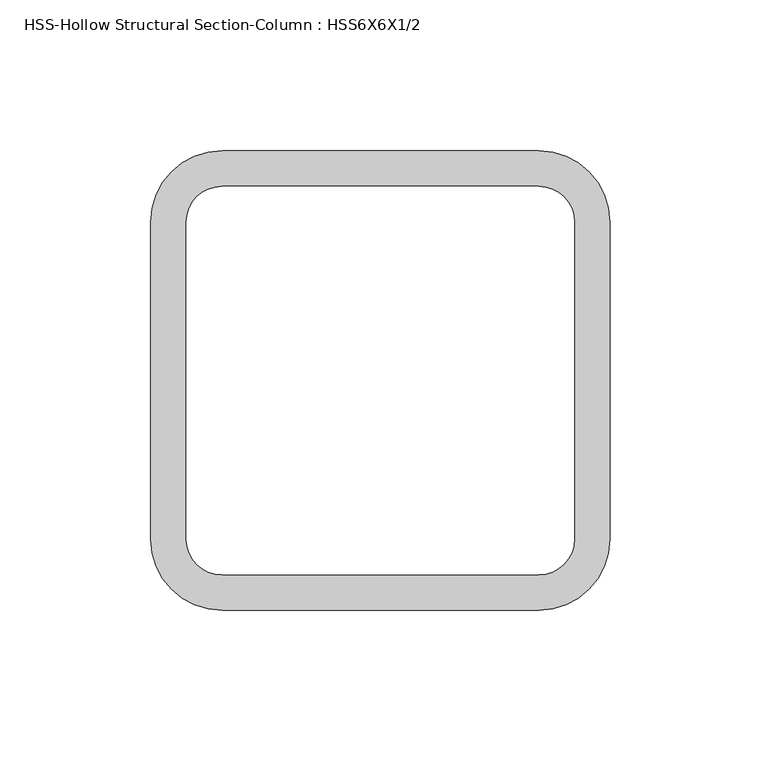
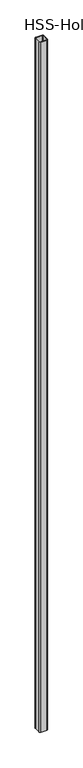
"""IFC4 building model written with IfcOpenShell, lengths in millimetres: column geometry, HSS-Hollow Structural Section-Column : HSS6X6X1/2."""

import ifcopenshell
import ifcopenshell.guid

model = None  # the IFC model being written
_history = None  # IfcOwnerHistory: only IFC2X3 demands one
_inside = {}  # id of a spatial element -> (the spatial element, [elements in it])
_under = {}  # id of a project, library or spatial element -> (it, [spatial elements below it])
_declared = {}  # id of a project -> (the project, [libraries it declares])
_typed = {}  # id of a type object -> (the type object, [elements of that type])
_made_of = {}  # id of a material, layer set ... -> (it, [elements and type objects made of it])


def new_model(schema):
    """Start an empty IFC model of exactly this schema.

    Asked for "IFC4X3", IfcOpenShell would pick the latest addendum, in which some entities
    have other attributes; the version numbers below select the first issue.
    IFC2X3 requires an IfcOwnerHistory on every rooted entity: one is made here for all.
    """
    global model, _history
    if schema == "IFC4X3":
        model = ifcopenshell.file(schema_version=(4, 3, 0, 0))
    else:
        model = ifcopenshell.file(schema=schema)
    _inside.clear()
    _under.clear()
    _declared.clear()
    _typed.clear()
    _made_of.clear()
    _history = None
    if model.schema == "IFC2X3":
        org = make("IfcOrganization", Name="unknown")
        user = make(
            "IfcPersonAndOrganization",
            ThePerson=make("IfcPerson", FamilyName="unknown"),
            TheOrganization=org,
        )
        app = make(
            "IfcApplication",
            ApplicationDeveloper=org,
            Version="unknown",
            ApplicationFullName="unknown",
            ApplicationIdentifier="unknown",
        )
        _history = make(
            "IfcOwnerHistory",
            OwningUser=user,
            OwningApplication=app,
            ChangeAction="ADDED",
            CreationDate=0,
        )
    return model


def make(cls, **values):
    """One entity of the class cls with the attributes given. An attribute that is None is left unset."""
    return model.create_entity(
        cls, **{name: value for name, value in values.items() if value is not None}
    )


def rooted(cls, **values):
    """An entity with a GlobalId (a new one), such as an element, a storey or a relation."""
    return make(cls, GlobalId=ifcopenshell.guid.new(), OwnerHistory=_history, **values)


def si_unit(unit_type, name, prefix=None):
    """IfcSIUnit, for example si_unit("LENGTHUNIT", "METRE", prefix="MILLI")."""
    return make("IfcSIUnit", UnitType=unit_type, Prefix=prefix, Name=name)


def assignment(units):
    """IfcUnitAssignment: the units of a project."""
    return None if units is None else make("IfcUnitAssignment", Units=units)


def point(xyz):
    """IfcCartesianPoint."""
    return None if xyz is None else make("IfcCartesianPoint", Coordinates=xyz)


def direction(xyz):
    """IfcDirection."""
    return None if xyz is None else make("IfcDirection", DirectionRatios=xyz)


def frame(location, z_axis=None, x_axis=None):
    """IfcAxis2Placement3D, a coordinate frame: its origin and axes. An axis left out is left unset."""
    return make(
        "IfcAxis2Placement3D",
        Location=point(location),
        Axis=direction(z_axis),
        RefDirection=direction(x_axis),
    )


def frame_2d(location, x_axis=None):
    """IfcAxis2Placement2D, a coordinate frame in the plane: its origin and x axis."""
    return make(
        "IfcAxis2Placement2D", Location=point(location), RefDirection=direction(x_axis)
    )


def origin():
    """The frame at (0, 0, 0) with its axes left unset."""
    return frame((0.0, 0.0, 0.0))


def place(relative_to, where):
    """IfcLocalPlacement: puts the frame where relative to a parent placement (None: the world)."""
    return make(
        "IfcLocalPlacement", PlacementRelTo=relative_to, RelativePlacement=where
    )


def context(
    kind, dimensions, precision=None, world=None, true_north=None, identifier=None
):
    """IfcGeometricRepresentationContext, for example the 3D "Model" context."""
    return make(
        "IfcGeometricRepresentationContext",
        ContextIdentifier=identifier,
        ContextType=kind,
        CoordinateSpaceDimension=dimensions,
        Precision=precision,
        WorldCoordinateSystem=world,
        TrueNorth=true_north,
    )


def project(units=None, contexts=None):
    """IfcProject with its units and contexts."""
    return rooted(
        "IfcProject",
        Name="project",
        RepresentationContexts=contexts,
        UnitsInContext=assignment(units),
    )


def spatial(cls, under=None, at=None, **own):
    """A site, building, storey or space (cls), placed at a placement, below another one or the project."""
    s = rooted(cls, ObjectPlacement=at, **own)
    if under is not None:
        _under.setdefault(under.id(), (under, []))[1].append(s)
    return s


def polyline(points):
    """IfcPolyline through the points."""
    return make("IfcPolyline", Points=[point(p) for p in points])


def circle_curve(where, radius):
    """IfcCircle in the frame where."""
    return make("IfcCircle", Position=where, Radius=radius)


def trimmed(basis, trim1, trim2, sense, master):
    """IfcTrimmedCurve: the piece of a basis curve between two trims."""
    return make(
        "IfcTrimmedCurve",
        BasisCurve=basis,
        Trim1=trim1,
        Trim2=trim2,
        SenseAgreement=sense,
        MasterRepresentation=master,
    )


def segment(curve, same_sense, transition):
    """IfcCompositeCurveSegment."""
    return make(
        "IfcCompositeCurveSegment",
        Transition=transition,
        SameSense=same_sense,
        ParentCurve=curve,
    )


def composite_curve(segments, self_intersect=None):
    """IfcCompositeCurve: segments joined end to end."""
    return make("IfcCompositeCurve", Segments=segments, SelfIntersect=self_intersect)


def outline(outer, holes=None, kind="AREA"):
    """IfcArbitraryClosedProfileDef: a profile drawn as a closed curve; with holes, ...WithVoids."""
    if holes is None:
        return make("IfcArbitraryClosedProfileDef", ProfileType=kind, OuterCurve=outer)
    return make(
        "IfcArbitraryProfileDefWithVoids",
        ProfileType=kind,
        OuterCurve=outer,
        InnerCurves=holes,
    )


def extrude(swept, where, along, depth):
    """IfcExtrudedAreaSolid: the profile swept, set in the frame where, extruded along a direction by depth."""
    return make(
        "IfcExtrudedAreaSolid",
        SweptArea=swept,
        Position=where,
        ExtrudedDirection=direction(along),
        Depth=depth,
    )


def shape(context_of_items, identifier, shape_type, items):
    """IfcShapeRepresentation: the items that make up one representation, for example the "Body"."""
    return make(
        "IfcShapeRepresentation",
        ContextOfItems=context_of_items,
        RepresentationIdentifier=identifier,
        RepresentationType=shape_type,
        Items=items,
    )


def source(mapping_origin, context_of_items, identifier, shape_type, items):
    """IfcRepresentationMap: a shape defined once, which mapped items show again and again."""
    return make(
        "IfcRepresentationMap",
        MappingOrigin=mapping_origin,
        MappedRepresentation=shape(context_of_items, identifier, shape_type, items),
    )


def transform(
    local_origin,
    x_axis=None,
    y_axis=None,
    z_axis=None,
    scale=None,
    scale2=None,
    scale3=None,
    uniform=True,
):
    """IfcCartesianTransformationOperator3D, or its non-uniform kind. x_axis, y_axis, z_axis: its Axis1, 2, 3."""
    if uniform:
        return make(
            "IfcCartesianTransformationOperator3D",
            Axis1=direction(x_axis),
            Axis2=direction(y_axis),
            LocalOrigin=point(local_origin),
            Scale=scale,
            Axis3=direction(z_axis),
        )
    return make(
        "IfcCartesianTransformationOperator3DnonUniform",
        Axis1=direction(x_axis),
        Axis2=direction(y_axis),
        LocalOrigin=point(local_origin),
        Scale=scale,
        Axis3=direction(z_axis),
        Scale2=scale2,
        Scale3=scale3,
    )


def mapped(mapping_source, mapping_target):
    """IfcMappedItem: shows the shape of a source again, moved by a transform."""
    return make(
        "IfcMappedItem", MappingSource=mapping_source, MappingTarget=mapping_target
    )


def made_of(thing, what):
    """Note that an element or type object is made of a material, layer set ...; save() writes the relation."""
    if what is not None:
        _made_of.setdefault(what.id(), (what, []))[1].append(thing)
    return thing


def element(
    cls,
    number,
    at=None,
    inside=None,
    cuts=None,
    type_object=None,
    material=None,
    context=None,
    identifier="Body",
    shape_type=None,
    held_by="IfcProductDefinitionShape",
    body=None,
    shapes=None,
    **own,
):
    """One element of the class cls, such as IfcWall. Its Tag is "e" and its number.

    at: its placement. inside: the storey or other place that contains it. cuts: it is an
    opening in that element (IfcRelVoidsElement). A single representation is given by context,
    identifier, shape_type and body (its items); several are given by shapes. held_by: the class
    of the entity that holds the representations. save() writes the other relations.
    """
    e = rooted(cls, Tag="e%d" % number, ObjectPlacement=at, **own)
    if body is not None:
        shapes = [shape(context, identifier, shape_type, body)]
    if shapes is not None:
        e.Representation = make(held_by, Representations=shapes)
    if inside is not None:
        _inside.setdefault(inside.id(), (inside, []))[1].append(e)
    if cuts is not None:
        rooted(
            "IfcRelVoidsElement", RelatingBuildingElement=cuts, RelatedOpeningElement=e
        )
    if type_object is not None:
        _typed.setdefault(type_object.id(), (type_object, []))[1].append(e)
    return made_of(e, material)


def aggregate(whole, parts):
    """IfcRelAggregates: a whole, such as a stair, and the parts it consists of."""
    return rooted("IfcRelAggregates", RelatingObject=whole, RelatedObjects=parts)


def save(model, path):
    """Write the relations noted so far, then the file.

    IfcRelAggregates (storeys below a building ...), IfcRelContainedInSpatialStructure (elements
    in a storey), IfcRelDefinesByType, IfcRelAssociatesMaterial and IfcRelDeclares: one each for
    every whole, place, type object, material and project.
    """
    for whole, parts in _under.values():
        aggregate(whole, parts)
    for where, things in _inside.values():
        rooted(
            "IfcRelContainedInSpatialStructure",
            RelatedElements=things,
            RelatingStructure=where,
        )
    for kind, things in _typed.values():
        rooted("IfcRelDefinesByType", RelatedObjects=things, RelatingType=kind)
    for what, things in _made_of.values():
        rooted("IfcRelAssociatesMaterial", RelatedObjects=things, RelatingMaterial=what)
    for by, libraries in _declared.values():
        rooted("IfcRelDeclares", RelatingContext=by, RelatedDefinitions=libraries)
    model.write(path)


def hss_hollow_structural_section_column_hss6x6x1_2_716acbd7(model_context):
    return source(origin(), model_context, "Body", "SweptSolid", [
        extrude(outline(composite_curve([segment(trimmed(circle_curve(frame_2d((52.578, 52.578)), 23.622), [point((52.578, 76.2))], [point((76.2, 52.578))], False, "CARTESIAN"), True, "CONTINUOUS"), segment(polyline([(76.2, 52.578), (76.2, -52.578)]), True, "CONTINUOUS"), segment(trimmed(circle_curve(frame_2d((52.578, -52.578)), 23.622), [point((76.2, -52.578))], [point((52.578, -76.2))], False, "CARTESIAN"), True, "CONTINUOUS"), segment(polyline([(52.578, -76.2), (-52.578, -76.2)]), True, "CONTINUOUS"), segment(trimmed(circle_curve(frame_2d((-52.578, -52.578)), 23.622), [point((-52.578, -76.2))], [point((-76.2, -52.578))], False, "CARTESIAN"), True, "CONTINUOUS"), segment(polyline([(-76.2, -52.578), (-76.2, 52.578)]), True, "CONTINUOUS"), segment(trimmed(circle_curve(frame_2d((-52.578, 52.578)), 23.622), [point((-76.2, 52.578))], [point((-52.578, 76.2))], False, "CARTESIAN"), True, "CONTINUOUS"), segment(polyline([(-52.578, 76.2), (52.578, 76.2)]), True, "CONTINUOUS")], self_intersect=False), holes=[composite_curve([segment(polyline([(52.578, 64.389), (-52.578, 64.389)]), True, "CONTINUOUS"), segment(trimmed(circle_curve(frame_2d((-52.578, 52.578)), 11.811), [point((-52.578, 64.389))], [point((-64.389, 52.578))], True, "CARTESIAN"), True, "CONTINUOUS"), segment(polyline([(-64.389, 52.578), (-64.389, -52.578)]), True, "CONTINUOUS"), segment(trimmed(circle_curve(frame_2d((-52.578, -52.578)), 11.811), [point((-64.389, -52.578))], [point((-52.578, -64.389))], True, "CARTESIAN"), True, "CONTINUOUS"), segment(polyline([(-52.578, -64.389), (52.578, -64.389)]), True, "CONTINUOUS"), segment(trimmed(circle_curve(frame_2d((52.578, -52.578)), 11.811), [point((52.578, -64.389))], [point((64.389, -52.578))], True, "CARTESIAN"), True, "CONTINUOUS"), segment(polyline([(64.389, -52.578), (64.389, 52.578)]), True, "CONTINUOUS"), segment(trimmed(circle_curve(frame_2d((52.578, 52.578)), 11.811), [point((64.389, 52.578))], [point((52.578, 64.389))], True, "CARTESIAN"), True, "CONTINUOUS")], self_intersect=False)]), frame((0.0, 0.0, -609.6), z_axis=(0.0, 0.0, 1.0), x_axis=(1.0, 0.0, 0.0)), (0.0, 0.0, 1.0), 13055.6),
    ])


if __name__ == "__main__":
    model = new_model("IFC4")
    model_context = context("Model", 3, world=origin())
    ifc_project = project(units=[si_unit("LENGTHUNIT", "METRE", prefix="MILLI")], contexts=[model_context])
    site = spatial("IfcSite", under=ifc_project)
    building = spatial("IfcBuilding", under=site)
    placement = place(None, origin())
    hss_hollow_structural_section_column_hss6x6x1_2_shape = hss_hollow_structural_section_column_hss6x6x1_2_716acbd7(model_context)
    element("IfcColumn", 1, ObjectType="HSS-Hollow Structural Section-Column : HSS6X6X1/2", at=placement, inside=building, context=model_context, shape_type="MappedRepresentation", body=[
        mapped(hss_hollow_structural_section_column_hss6x6x1_2_shape, transform((0.0, 0.0, 0.0), x_axis=(1.0, 0.0, 0.0), y_axis=(0.0, 1.0, 0.0), z_axis=(0.0, 0.0, 1.0))),
    ])
    save(model, "model.ifc")

# Revit data of these elements
# Type "HSS-Hollow Structural Section-Column : HSS6X6X1/2"
#   Assembly Code = "B10"
#   Shape = "Square"
#   W = 35.1
#   Ht = 0' - 6"
#   b = 0' - 6"
#   kr = 0' - 0.93"
#   t = 0' - 0.465"
#   A = 0.0676389 SF
#   Structural Material [instance default] = Steel ASTM A500, Grade B, Rectangular and Square
# Element 1 (IfcColumn, "HSS-Hollow Structural Section-Column : HSS6X6X1/2")
#   Materials on its faces: "Steel ASTM A500, Grade B, Rectangular and Square"
# Materials
#   "Steel ASTM A500, Grade B, Rectangular and Square": class "Metal", colour RGB 199 199 199, transparency 0, Description = "Carbon steel", Cost = 0
